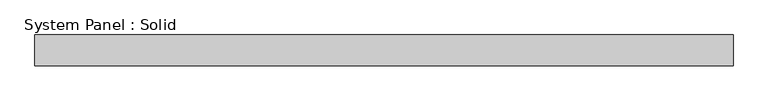
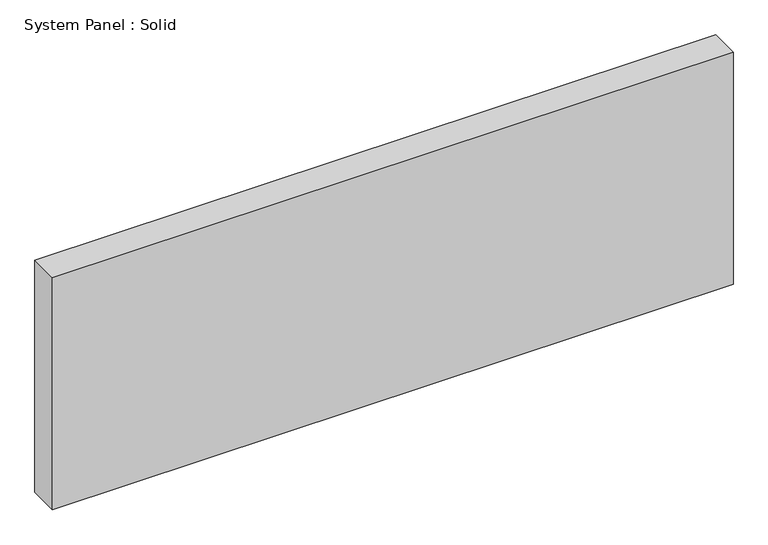
"""IFC4 building model written with IfcOpenShell, lengths in millimetres: plate geometry, System Panel : Solid."""

import ifcopenshell
import ifcopenshell.guid

model = None  # the IFC model being written
_history = None  # IfcOwnerHistory: only IFC2X3 demands one
_inside = {}  # id of a spatial element -> (the spatial element, [elements in it])
_under = {}  # id of a project, library or spatial element -> (it, [spatial elements below it])
_declared = {}  # id of a project -> (the project, [libraries it declares])
_typed = {}  # id of a type object -> (the type object, [elements of that type])
_made_of = {}  # id of a material, layer set ... -> (it, [elements and type objects made of it])


def new_model(schema):
    """Start an empty IFC model of exactly this schema.

    Asked for "IFC4X3", IfcOpenShell would pick the latest addendum, in which some entities
    have other attributes; the version numbers below select the first issue.
    IFC2X3 requires an IfcOwnerHistory on every rooted entity: one is made here for all.
    """
    global model, _history
    if schema == "IFC4X3":
        model = ifcopenshell.file(schema_version=(4, 3, 0, 0))
    else:
        model = ifcopenshell.file(schema=schema)
    _inside.clear()
    _under.clear()
    _declared.clear()
    _typed.clear()
    _made_of.clear()
    _history = None
    if model.schema == "IFC2X3":
        org = make("IfcOrganization", Name="unknown")
        user = make(
            "IfcPersonAndOrganization",
            ThePerson=make("IfcPerson", FamilyName="unknown"),
            TheOrganization=org,
        )
        app = make(
            "IfcApplication",
            ApplicationDeveloper=org,
            Version="unknown",
            ApplicationFullName="unknown",
            ApplicationIdentifier="unknown",
        )
        _history = make(
            "IfcOwnerHistory",
            OwningUser=user,
            OwningApplication=app,
            ChangeAction="ADDED",
            CreationDate=0,
        )
    return model


def make(cls, **values):
    """One entity of the class cls with the attributes given. An attribute that is None is left unset."""
    return model.create_entity(
        cls, **{name: value for name, value in values.items() if value is not None}
    )


def rooted(cls, **values):
    """An entity with a GlobalId (a new one), such as an element, a storey or a relation."""
    return make(cls, GlobalId=ifcopenshell.guid.new(), OwnerHistory=_history, **values)


def si_unit(unit_type, name, prefix=None):
    """IfcSIUnit, for example si_unit("LENGTHUNIT", "METRE", prefix="MILLI")."""
    return make("IfcSIUnit", UnitType=unit_type, Prefix=prefix, Name=name)


def assignment(units):
    """IfcUnitAssignment: the units of a project."""
    return None if units is None else make("IfcUnitAssignment", Units=units)


def point(xyz):
    """IfcCartesianPoint."""
    return None if xyz is None else make("IfcCartesianPoint", Coordinates=xyz)


def direction(xyz):
    """IfcDirection."""
    return None if xyz is None else make("IfcDirection", DirectionRatios=xyz)


def frame(location, z_axis=None, x_axis=None):
    """IfcAxis2Placement3D, a coordinate frame: its origin and axes. An axis left out is left unset."""
    return make(
        "IfcAxis2Placement3D",
        Location=point(location),
        Axis=direction(z_axis),
        RefDirection=direction(x_axis),
    )


def origin():
    """The frame at (0, 0, 0) with its axes left unset."""
    return frame((0.0, 0.0, 0.0))


def origin_with_axes():
    """The frame at (0, 0, 0) with the z axis (0, 0, 1) and the x axis (1, 0, 0) written out."""
    return frame((0.0, 0.0, 0.0), z_axis=(0.0, 0.0, 1.0), x_axis=(1.0, 0.0, 0.0))


def place(relative_to, where):
    """IfcLocalPlacement: puts the frame where relative to a parent placement (None: the world)."""
    return make(
        "IfcLocalPlacement", PlacementRelTo=relative_to, RelativePlacement=where
    )


def context(
    kind, dimensions, precision=None, world=None, true_north=None, identifier=None
):
    """IfcGeometricRepresentationContext, for example the 3D "Model" context."""
    return make(
        "IfcGeometricRepresentationContext",
        ContextIdentifier=identifier,
        ContextType=kind,
        CoordinateSpaceDimension=dimensions,
        Precision=precision,
        WorldCoordinateSystem=world,
        TrueNorth=true_north,
    )


def project(units=None, contexts=None):
    """IfcProject with its units and contexts."""
    return rooted(
        "IfcProject",
        Name="project",
        RepresentationContexts=contexts,
        UnitsInContext=assignment(units),
    )


def spatial(cls, under=None, at=None, **own):
    """A site, building, storey or space (cls), placed at a placement, below another one or the project."""
    s = rooted(cls, ObjectPlacement=at, **own)
    if under is not None:
        _under.setdefault(under.id(), (under, []))[1].append(s)
    return s


def polyline(points):
    """IfcPolyline through the points."""
    return make("IfcPolyline", Points=[point(p) for p in points])


def outline(outer, holes=None, kind="AREA"):
    """IfcArbitraryClosedProfileDef: a profile drawn as a closed curve; with holes, ...WithVoids."""
    if holes is None:
        return make("IfcArbitraryClosedProfileDef", ProfileType=kind, OuterCurve=outer)
    return make(
        "IfcArbitraryProfileDefWithVoids",
        ProfileType=kind,
        OuterCurve=outer,
        InnerCurves=holes,
    )


def extrude(swept, where, along, depth):
    """IfcExtrudedAreaSolid: the profile swept, set in the frame where, extruded along a direction by depth."""
    return make(
        "IfcExtrudedAreaSolid",
        SweptArea=swept,
        Position=where,
        ExtrudedDirection=direction(along),
        Depth=depth,
    )


def shape(context_of_items, identifier, shape_type, items):
    """IfcShapeRepresentation: the items that make up one representation, for example the "Body"."""
    return make(
        "IfcShapeRepresentation",
        ContextOfItems=context_of_items,
        RepresentationIdentifier=identifier,
        RepresentationType=shape_type,
        Items=items,
    )


def source(mapping_origin, context_of_items, identifier, shape_type, items):
    """IfcRepresentationMap: a shape defined once, which mapped items show again and again."""
    return make(
        "IfcRepresentationMap",
        MappingOrigin=mapping_origin,
        MappedRepresentation=shape(context_of_items, identifier, shape_type, items),
    )


def transform(
    local_origin,
    x_axis=None,
    y_axis=None,
    z_axis=None,
    scale=None,
    scale2=None,
    scale3=None,
    uniform=True,
):
    """IfcCartesianTransformationOperator3D, or its non-uniform kind. x_axis, y_axis, z_axis: its Axis1, 2, 3."""
    if uniform:
        return make(
            "IfcCartesianTransformationOperator3D",
            Axis1=direction(x_axis),
            Axis2=direction(y_axis),
            LocalOrigin=point(local_origin),
            Scale=scale,
            Axis3=direction(z_axis),
        )
    return make(
        "IfcCartesianTransformationOperator3DnonUniform",
        Axis1=direction(x_axis),
        Axis2=direction(y_axis),
        LocalOrigin=point(local_origin),
        Scale=scale,
        Axis3=direction(z_axis),
        Scale2=scale2,
        Scale3=scale3,
    )


def mapped(mapping_source, mapping_target):
    """IfcMappedItem: shows the shape of a source again, moved by a transform."""
    return make(
        "IfcMappedItem", MappingSource=mapping_source, MappingTarget=mapping_target
    )


def made_of(thing, what):
    """Note that an element or type object is made of a material, layer set ...; save() writes the relation."""
    if what is not None:
        _made_of.setdefault(what.id(), (what, []))[1].append(thing)
    return thing


def element(
    cls,
    number,
    at=None,
    inside=None,
    cuts=None,
    type_object=None,
    material=None,
    context=None,
    identifier="Body",
    shape_type=None,
    held_by="IfcProductDefinitionShape",
    body=None,
    shapes=None,
    **own,
):
    """One element of the class cls, such as IfcWall. Its Tag is "e" and its number.

    at: its placement. inside: the storey or other place that contains it. cuts: it is an
    opening in that element (IfcRelVoidsElement). A single representation is given by context,
    identifier, shape_type and body (its items); several are given by shapes. held_by: the class
    of the entity that holds the representations. save() writes the other relations.
    """
    e = rooted(cls, Tag="e%d" % number, ObjectPlacement=at, **own)
    if body is not None:
        shapes = [shape(context, identifier, shape_type, body)]
    if shapes is not None:
        e.Representation = make(held_by, Representations=shapes)
    if inside is not None:
        _inside.setdefault(inside.id(), (inside, []))[1].append(e)
    if cuts is not None:
        rooted(
            "IfcRelVoidsElement", RelatingBuildingElement=cuts, RelatedOpeningElement=e
        )
    if type_object is not None:
        _typed.setdefault(type_object.id(), (type_object, []))[1].append(e)
    return made_of(e, material)


def aggregate(whole, parts):
    """IfcRelAggregates: a whole, such as a stair, and the parts it consists of."""
    return rooted("IfcRelAggregates", RelatingObject=whole, RelatedObjects=parts)


def save(model, path):
    """Write the relations noted so far, then the file.

    IfcRelAggregates (storeys below a building ...), IfcRelContainedInSpatialStructure (elements
    in a storey), IfcRelDefinesByType, IfcRelAssociatesMaterial and IfcRelDeclares: one each for
    every whole, place, type object, material and project.
    """
    for whole, parts in _under.values():
        aggregate(whole, parts)
    for where, things in _inside.values():
        rooted(
            "IfcRelContainedInSpatialStructure",
            RelatedElements=things,
            RelatingStructure=where,
        )
    for kind, things in _typed.values():
        rooted("IfcRelDefinesByType", RelatedObjects=things, RelatingType=kind)
    for what, things in _made_of.values():
        rooted("IfcRelAssociatesMaterial", RelatedObjects=things, RelatingMaterial=what)
    for by, libraries in _declared.values():
        rooted("IfcRelDeclares", RelatingContext=by, RelatedDefinitions=libraries)
    model.write(path)


def system_panel_solid_4932440a(model_context):
    return source(origin(), model_context, "Body", "SweptSolid", [
        extrude(outline(polyline([(713.3166666, -19.05), (-713.3166666, -19.05), (-713.3166666, 44.45), (713.3166666, 44.45), (713.3166666, -19.05)])), origin_with_axes(), (0.0, 0.0, 1.0), 514.35),
    ])


if __name__ == "__main__":
    model = new_model("IFC4")
    model_context = context("Model", 3, world=origin())
    ifc_project = project(units=[si_unit("LENGTHUNIT", "METRE", prefix="MILLI")], contexts=[model_context])
    site = spatial("IfcSite", under=ifc_project)
    building = spatial("IfcBuilding", under=site)
    placement = place(None, origin())
    system_panel_solid_shape = system_panel_solid_4932440a(model_context)
    element("IfcPlate", 1, ObjectType="System Panel : Solid", at=placement, inside=building, context=model_context, shape_type="MappedRepresentation", body=[
        mapped(system_panel_solid_shape, transform((0.0, 0.0, 0.0), x_axis=(1.0, 0.0, 0.0), y_axis=(0.0, 1.0, 0.0), z_axis=(0.0, 0.0, 1.0))),
    ])
    save(model, "model.ifc")

# Revit data of these elements
# Type "System Panel : Solid"
#   Construction Type Id = "MDOOR"
#   Analytic Construction = "Metal"
#   Visual Light Transmittance = 0
#   Solar Heat Gain Coefficient = 0
#   Heat Transfer Coefficient (U) = 0.651978 BTU/(h·ft²·°F)
#   Define Thermal Properties by = 1
# Element 1 (IfcPlate, "System Panel : Solid")
#   Materials on its faces: "Default"
# Materials
#   "Default": class "Miscellaneous", colour RGB 127 127 127, transparency 0, Cost = 0
